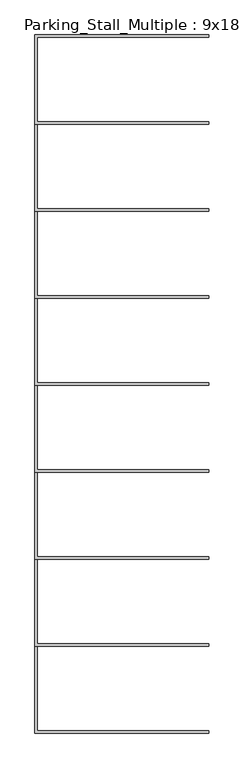
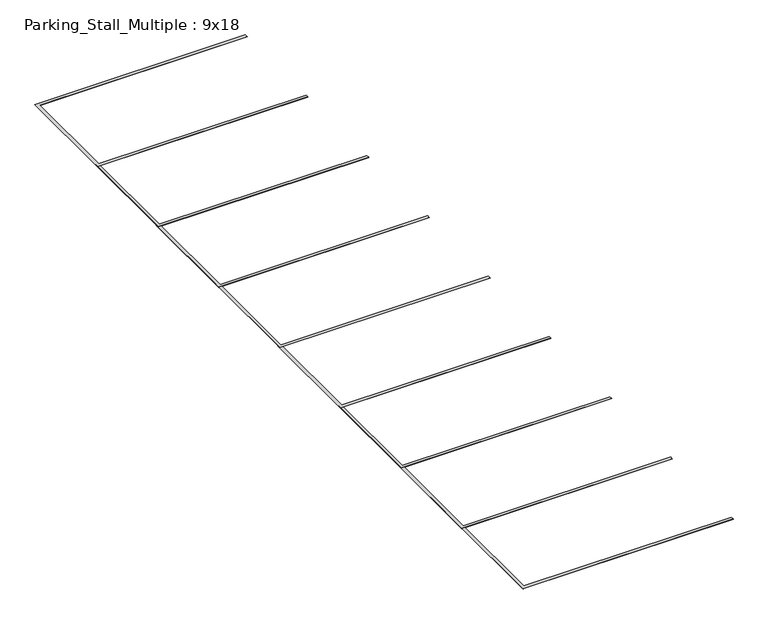
"""IFC4 building model written with IfcOpenShell, lengths in millimetres: proxy geometry, Parking_Stall_Multiple : 9x18."""

from ifc_helpers import new_model, si_unit, origin, origin_with_axes, place, context, project, spatial, polyline, outline, extrude, source, transform, mapped, element, save


def parking_stall_multiple_9x18_41294f2a(model_context):
    return source(origin(), model_context, "Body", "SweptSolid", [
        extrude(outline(polyline([(5486.4, 19202.4), (0.0, 19202.4), (0.0, 22021.8), (5486.4, 22021.8), (5486.4, 21945.6), (76.2, 21945.6), (76.2, 19278.6), (5486.4, 19278.6), (5486.4, 19202.4)])), origin_with_axes(), (0.0, 0.0, 1.0), 6.35),
        extrude(outline(polyline([(5486.4, 16459.2), (0.0, 16459.2), (0.0, 19278.6), (5486.4, 19278.6), (5486.4, 19202.4), (76.2, 19202.4), (76.2, 16535.4), (5486.4, 16535.4), (5486.4, 16459.2)])), origin_with_axes(), (0.0, 0.0, 1.0), 6.35),
        extrude(outline(polyline([(5486.4, 13716.0), (0.0, 13716.0), (0.0, 16535.4), (5486.4, 16535.4), (5486.4, 16459.2), (76.2, 16459.2), (76.2, 13792.2), (5486.4, 13792.2), (5486.4, 13716.0)])), origin_with_axes(), (0.0, 0.0, 1.0), 6.35),
        extrude(outline(polyline([(5486.4, 10972.8), (0.0, 10972.8), (0.0, 13792.2), (5486.4, 13792.2), (5486.4, 13716.0), (76.2, 13716.0), (76.2, 11049.0), (5486.4, 11049.0), (5486.4, 10972.8)])), origin_with_axes(), (0.0, 0.0, 1.0), 6.35),
        extrude(outline(polyline([(5486.4, 8229.6), (0.0, 8229.6), (0.0, 11049.0), (5486.4, 11049.0), (5486.4, 10972.8), (76.2, 10972.8), (76.2, 8305.8), (5486.4, 8305.8), (5486.4, 8229.6)])), origin_with_axes(), (0.0, 0.0, 1.0), 6.35),
        extrude(outline(polyline([(5486.4, 5486.4), (0.0, 5486.4), (0.0, 8305.8), (5486.4, 8305.8), (5486.4, 8229.6), (76.2, 8229.6), (76.2, 5562.6), (5486.4, 5562.6), (5486.4, 5486.4)])), origin_with_axes(), (0.0, 0.0, 1.0), 6.35),
        extrude(outline(polyline([(5486.4, 2743.2), (0.0, 2743.2), (0.0, 5562.6), (5486.4, 5562.6), (5486.4, 5486.4), (76.2, 5486.4), (76.2, 2819.4), (5486.4, 2819.4), (5486.4, 2743.2)])), origin_with_axes(), (0.0, 0.0, 1.0), 6.35),
        extrude(outline(polyline([(5486.4, 0.0), (0.0, 0.0), (0.0, 2819.4), (5486.4, 2819.4), (5486.4, 2743.2), (76.2, 2743.2), (76.2, 76.2), (5486.4, 76.2), (5486.4, 0.0)])), origin_with_axes(), (0.0, 0.0, 1.0), 6.35),
    ])


if __name__ == "__main__":
    model = new_model("IFC4")
    model_context = context("Model", 3, world=origin())
    ifc_project = project(units=[si_unit("LENGTHUNIT", "METRE", prefix="MILLI")], contexts=[model_context])
    site = spatial("IfcSite", under=ifc_project)
    building = spatial("IfcBuilding", under=site)
    placement = place(None, origin())
    parking_stall_multiple_9x18_shape = parking_stall_multiple_9x18_41294f2a(model_context)
    element("IfcBuildingElementProxy", 1, Name="Parking_Stall_Multiple : 9x18", ObjectType="Parking_Stall_Multiple : 9x18", at=placement, inside=building, context=model_context, shape_type="MappedRepresentation", body=[
        mapped(parking_stall_multiple_9x18_shape, transform((0.0, 0.0, 0.0), x_axis=(1.0, 0.0, 0.0), y_axis=(0.0, 1.0, 0.0), z_axis=(0.0, 0.0, 1.0))),
    ])
    save(model, "model.ifc")

# Revit data of these elements
# Type "Parking_Stall_Multiple : 9x18"
#   Parking_Width_M = 9' - 0"
#   Parking_Run_Length [instance default] = 65' - 0"
#   Parking_Line_Width = 0' - 3"
#   Parking_Length_M = 18' - 0"
#   Single_Parking_Visibility [instance default] = no
#   Parking_ADA_Symbol = no
#   ParkingUnitsArray [instance default] = 7
#   ParkingUnits [instance default] = 7
#   Multiple_Parking_Visibility [instance default] = yes
#   Parking_Line_Material = ADA VAN ACCESSIBLE STALL
# Element 1 (IfcBuildingElementProxy, "Parking_Stall_Multiple : 9x18")
#   Parking_Run_Length = 70' - 11.05727"
#   ParkingUnitsArray = 8
#   ParkingUnits = 8
#   Materials on its faces: "ADA VAN ACCESSIBLE STALL"
# Materials
#   "ADA VAN ACCESSIBLE STALL": class "Paint", colour RGB 255 255 255, transparency 0, Cost = 0
